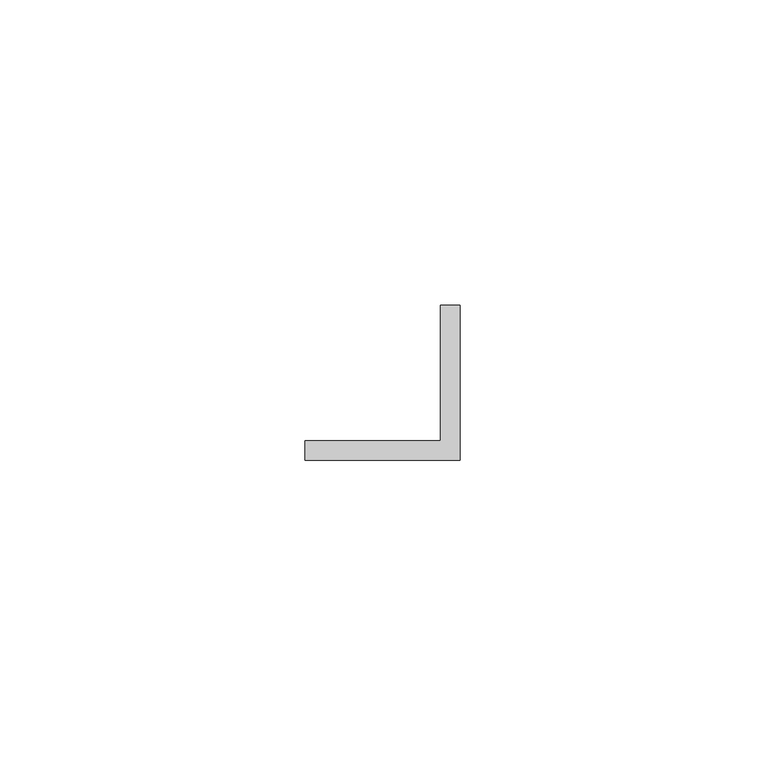
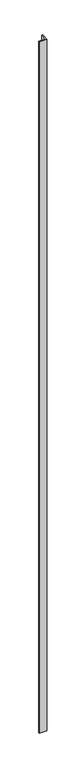
"""IFC4 building model written with IfcOpenShell, lengths in millimetres: proxy geometry, Lower profile:Lower profile:1:Lower profile:1 : Lower profile:Lower profile:300380:301093:Lower profile:1:Lower profile:1 : Lower profile:Lower profile:300380:301093 : Lower profile:Lower profile:1:Lower profile:1 : Lower profile:Lower profile:300380:301093:6 : Lower profile:Lower profile:1:Lower profile:1 : Lower profile:Lower profile:300380:301093:Lower profile:1:Lower profile:1 : Lower profile:Lower profile:300380:301093 : Lower profile:Lower profile:1:Lower profile:1 : Lower profile:Lower profile:300380:301093:300247."""

from ifc_helpers import new_model, si_unit, frame, origin, place, context, project, spatial, polyline, outline, extrude, source, transform, mapped, element, save


def generic_models_36ebcf0e(model_context):
    return source(origin(), model_context, "Body", "SweptSolid", [
        extrude(outline(polyline([(593738.0867239, -578772.0913841), (593738.0867239, -578797.4913841), (593712.6867239, -578797.4913841), (593712.6867239, -578794.268987), (593734.9117239, -578794.268987), (593734.9117239, -578772.0913841), (593738.0867239, -578772.0913841)])), frame((0.0, 0.0, 44.45), z_axis=(0.0, 0.0, 1.0), x_axis=(1.0, 0.0, 0.0)), (0.0, 0.0, 1.0), 2444.75),
    ])


if __name__ == "__main__":
    model = new_model("IFC4")
    model_context = context("Model", 3, world=origin())
    ifc_project = project(units=[si_unit("LENGTHUNIT", "METRE", prefix="MILLI")], contexts=[model_context])
    site = spatial("IfcSite", under=ifc_project)
    building = spatial("IfcBuilding", under=site)
    placement = place(None, origin())
    generic_models_shape = generic_models_36ebcf0e(model_context)
    element("IfcBuildingElementProxy", 1, Name="Lower profile:Lower profile:1:Lower profile:1 : Lower profile:Lower profile:300380:301093:Lower profile:1:Lower profile:1 : Lower profile:Lower profile:300380:301093 : Lower profile:Lower profile:1:Lower profile:1 : Lower profile:Lower profile:300380:301093:6 : Lower profile:Lower profile:1:Lower profile:1 : Lower profile:Lower profile:300380:301093:Lower profile:1:Lower profile:1 : Lower profile:Lower profile:300380:301093 : Lower profile:Lower profile:1:Lower profile:1 : Lower profile:Lower profile:300380:301093:300247", ObjectType="Lower profile:Lower profile:1:Lower profile:1 : Lower profile:Lower profile:300380:301093:Lower profile:1:Lower profile:1 : Lower profile:Lower profile:300380:301093 : Lower profile:Lower profile:1:Lower profile:1 : Lower profile:Lower profile:300380:301093:6 : Lower profile:Lower profile:1:Lower profile:1 : Lower profile:Lower profile:300380:301093:Lower profile:1:Lower profile:1 : Lower profile:Lower profile:300380:301093 : Lower profile:Lower profile:1:Lower profile:1 : Lower profile:Lower profile:300380:301093:300247", at=placement, inside=building, context=model_context, shape_type="MappedRepresentation", body=[
        mapped(generic_models_shape, transform((0.0, 0.0, 0.0), x_axis=(1.0, 0.0, 0.0), y_axis=(0.0, 1.0, 0.0), z_axis=(0.0, 0.0, 1.0))),
    ])
    save(model, "model.ifc")

# Revit data of these elements
# Type "Lower profile:Lower profile:1:Lower profile:1 : Lower profile:Lower profile:300380:301093:Lower profile:1:Lower profile:1 : Lower profile:Lower profile:300380:301093 : Lower profile:Lower profile:1:Lower profile:1 : Lower profile:Lower profile:300380:301093:6 : Lower profile:Lower profile:1:Lower profile:1 : Lower profile:Lower profile:300380:301093:Lower profile:1:Lower profile:1 : Lower profile:Lower profile:300380:301093 : Lower profile:Lower profile:1:Lower profile:1 : Lower profile:Lower profile:300380:301093:300247"
#   NameOverride = "Lower profile:Lower profile:1:Lower profile:1 : Lower profile:Lower profile:300380:301093:Lower profile:1:Lower profile:1 : Lower profile:Lower profile:300380:301093 : Lower profile:Lower profile:1:Lower profile:1 : Lower profile:Lower profile:300380:301093:300247"
#   ObjectTypeOverride = "Lower profile:1:Lower profile:1 : Lower profile:Lower profile:300380:301093 : Lower profile:Lower profile:1:Lower profile:1 : Lower profile:Lower profile:300380:301093"
#   Reference = "Lower profile"
#   Tag = "300247"
# Element 1 (IfcBuildingElementProxy, "Lower profile:Lower profile:1:Lower profile:1 : Lower profile:Lower profile:300380:301093:Lower profile:1:Lower profile:1 : Lower profile:Lower profile:300380:301093 : Lower profile:Lower profile:1:Lower profile:1 : Lower profile:Lower profile:300380:301093:6 : Lower profile:Lower profile:1:Lower profile:1 : Lower profile:Lower profile:300380:301093:Lower profile:1:Lower profile:1 : Lower profile:Lower profile:300380:301093 : Lower profile:Lower profile:1:Lower profile:1 : Lower profile:Lower profile:300380:301093:300247")
#   Materials on its faces: "1\" X 1\" X 1/8\" ALUM. ANGLE"
# Materials
#   "1\" X 1\" X 1/8\" ALUM. ANGLE": class "Metal", colour RGB 244 244 244, transparency 0, Description = "Aluminum 6061", Cost = 0
